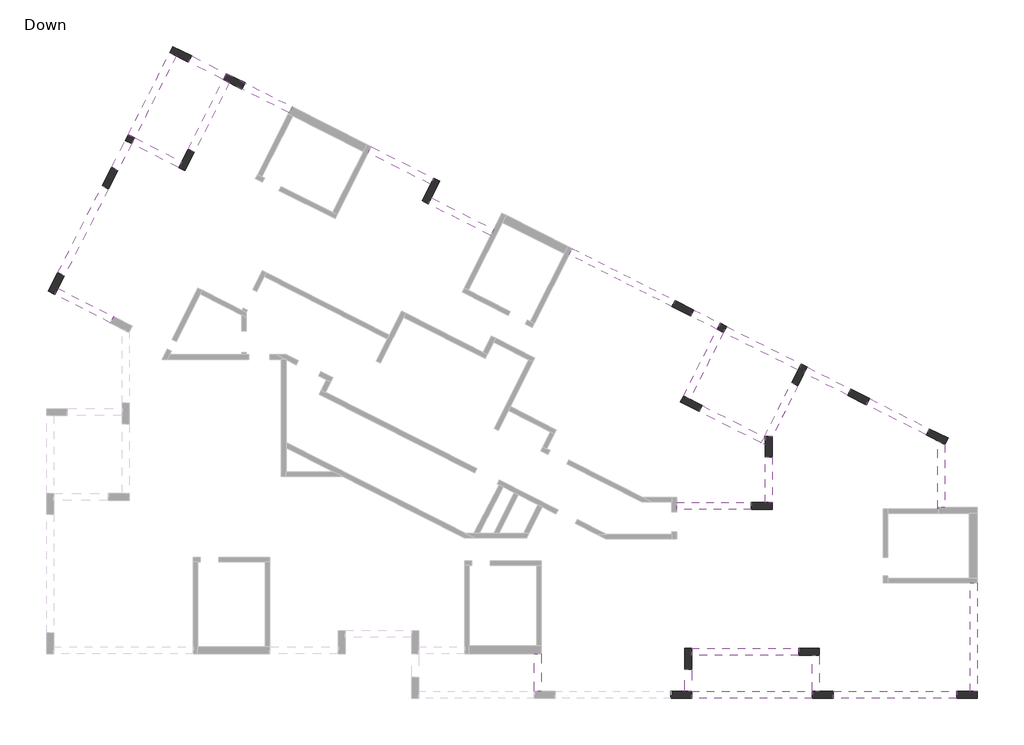
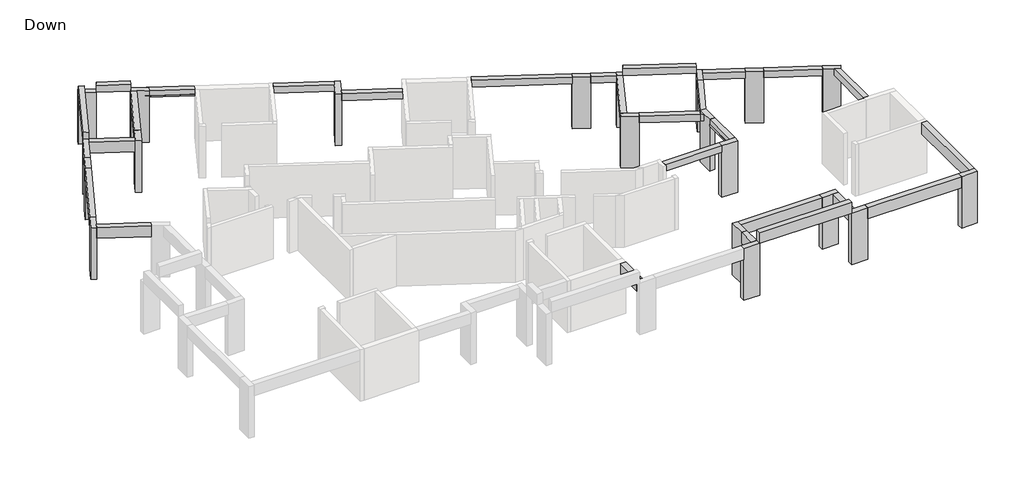
# One storey, part 3 of 3: 28 beams, 20 columns.
# Revit data of these elements (continued)
# Element 42 (IfcColumn, "Concrete Rectengular Column : 30/90") (continued)
#   Mark = "C23"
#   SOFiSTiK_AMG_Comments = ""
#   SOFiSTiK_AMG_Scheduled = yes
#   SOFiSTiK_AMG_Adjusted = yes
#   Structural Material = Concrete
#   Phase Created = New Construction
#   Materials on its faces: "Concrete"
# Element 43 (IfcColumn, "Concrete Rectengular Column : 30/90")
#   Comments = ""
#   Mark = "C24"
#   SOFiSTiK_AMG_Comments = ""
#   SOFiSTiK_AMG_Scheduled = yes
#   SOFiSTiK_AMG_Adjusted = yes
#   Structural Material = Concrete
#   Phase Created = New Construction
#   Materials on its faces: "Concrete"
# Element 44 (IfcColumn, "Concrete Rectengular Column : 30/90")
#   Comments = ""
#   Mark = "C25"
#   SOFiSTiK_AMG_Comments = ""
#   SOFiSTiK_AMG_Scheduled = yes
#   SOFiSTiK_AMG_Adjusted = yes
#   Structural Material = Concrete
#   Phase Created = New Construction
#   Materials on its faces: "Concrete"
# Element 45 (IfcColumn, "Concrete Rectengular Column : 30/90")
#   Comments = ""
#   Mark = "C26"
#   SOFiSTiK_AMG_Comments = ""
#   SOFiSTiK_AMG_Scheduled = yes
#   SOFiSTiK_AMG_Adjusted = yes
#   Structural Material = Concrete
#   Phase Created = New Construction
#   Materials on its faces: "Concrete"
# Element 46 (IfcColumn, "Concrete Rectengular Column : 30/90")
#   Comments = ""
#   Mark = "C28"
#   SOFiSTiK_AMG_Comments = ""
#   SOFiSTiK_AMG_Scheduled = yes
#   SOFiSTiK_AMG_Adjusted = yes
#   Structural Material = Concrete
#   Phase Created = New Construction
#   Materials on its faces: "Concrete"
# Element 47 (IfcColumn, "Concrete Rectengular Column : 30/90")
#   Comments = ""
#   Mark = "C29"
#   SOFiSTiK_AMG_Comments = ""
#   SOFiSTiK_AMG_Scheduled = yes
#   SOFiSTiK_AMG_Adjusted = yes
#   Structural Material = Concrete
#   Phase Created = New Construction
#   Materials on its faces: "Concrete"
# Element 48 (IfcColumn, "Concrete Rectengular Column : 30/90")
#   Comments = ""
#   Mark = "C30"
#   SOFiSTiK_AMG_Comments = ""
#   SOFiSTiK_AMG_Scheduled = yes
#   SOFiSTiK_AMG_Adjusted = yes
#   Structural Material = Concrete
#   Phase Created = New Construction
#   Materials on its faces: "Concrete"
# Materials
#   "Concrete": class "Concrete", colour RGB 192 192 192, transparency 0, Keynote = "01000", Description = "Cast-in-place concrete", Cost = 0
